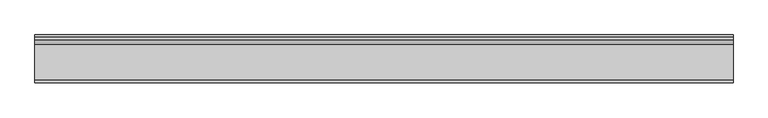
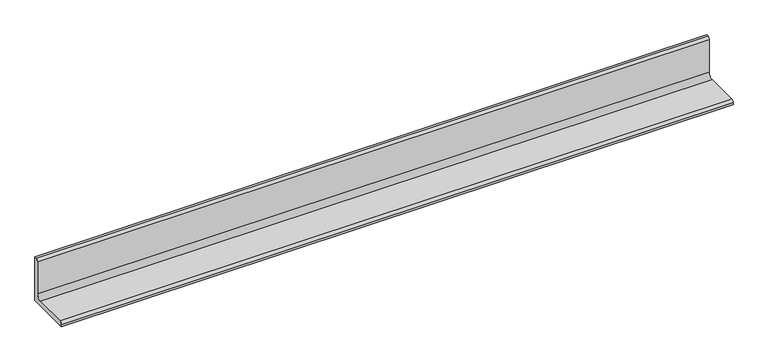
"""IFC4 building model written with IfcOpenShell, lengths in millimetres: beam geometry, NLRS_28_SF_LIB_stalen ligger hoekprofiel gelijkzijdig-AV-MMBS-SRP_gen_rsf : stalen ligger gelijkzijdig hoekprofiel LEQU_gen__150x150x15."""

from ifc_helpers import new_model, si_unit, point, frame, frame_2d, origin, place, context, project, spatial, polyline, circle_curve, trimmed, segment, composite_curve, outline, extrude, source, transform, mapped, element, save


def beam_a9a0024c(model_context):
    return source(origin(), model_context, "Body", "SweptSolid", [
        extrude(outline(composite_curve([segment(polyline([(42.5, -42.5), (-107.5, -42.5), (-107.5, -35.5)]), True, "CONTINUOUS"), segment(trimmed(circle_curve(frame_2d((-99.5, -35.5)), 8.0), [point((-107.5, -35.5))], [point((-99.5, -27.5))], False, "CARTESIAN"), True, "CONTINUOUS"), segment(polyline([(-99.5, -27.5), (11.5, -27.5)]), True, "CONTINUOUS"), segment(trimmed(circle_curve(frame_2d((11.5, -11.5)), 16.0), [point((11.5, -27.5))], [point((27.5, -11.5))], True, "CARTESIAN"), True, "CONTINUOUS"), segment(polyline([(27.5, -11.5), (27.5, 99.5)]), True, "CONTINUOUS"), segment(trimmed(circle_curve(frame_2d((35.5, 99.5)), 8.0), [point((27.5, 99.5))], [point((35.5, 107.5))], False, "CARTESIAN"), True, "CONTINUOUS"), segment(polyline([(35.5, 107.5), (42.5, 107.5), (42.5, -42.5)]), True, "CONTINUOUS")], self_intersect=False)), frame((-1095.0, 0.0, 0.0), z_axis=(1.0, 0.0, 0.0), x_axis=(0.0, 1.0, 0.0)), (0.0, 0.0, 1.0), 2190.0),
    ])


if __name__ == "__main__":
    model = new_model("IFC4")
    model_context = context("Model", 3, world=origin())
    ifc_project = project(units=[si_unit("LENGTHUNIT", "METRE", prefix="MILLI")], contexts=[model_context])
    site = spatial("IfcSite", under=ifc_project)
    building = spatial("IfcBuilding", under=site)
    placement = place(None, origin())
    beam_shape = beam_a9a0024c(model_context)
    element("IfcBeam", 1, ObjectType="NLRS_28_SF_LIB_stalen ligger hoekprofiel gelijkzijdig-AV-MMBS-SRP_gen_rsf : stalen ligger gelijkzijdig hoekprofiel LEQU_gen__150x150x15", at=placement, inside=building, context=model_context, shape_type="MappedRepresentation", body=[
        mapped(beam_shape, transform((0.0, 0.0, 0.0), x_axis=(1.0, 0.0, 0.0), y_axis=(0.0, 1.0, 0.0), z_axis=(0.0, 0.0, 1.0))),
    ])
    save(model, "model.ifc")

# Revit data of these elements
# Type "NLRS_28_SF_LIB_stalen ligger hoekprofiel gelijkzijdig-AV-MMBS-SRP_gen_rsf : stalen ligger gelijkzijdig hoekprofiel LEQU_gen__150x150x15"
#   Type IfcGUID = "2CEqVLPNH8KRN7ghwV3a1U"
#   IfcExportAs = "IfcBeamType"
#   Type Comments = "L150x150x15"
#   Model = " "
#   Manufacturer = " "
#   Fire Rating = " "
#   Description = "stalen ligger L150x150x15"
#   Assembly Code = "28.11"
#   vz = 107.5 mm
#   vy = 107.5 mm
#   tw = 15 mm
#   tf = 15 mm
#   ri = 8 mm
#   ra = 16 mm
#   d = 150 mm
#   bf = 150 mm
#   NLRS_C_lengte [instance default] = 1524 mm
#   Length [instance default] = 1524 mm
#   Structural Material = NLRS_h2_staal_gen_rsf
#   Keynote = ""
# Element 1 (IfcBeam, "NLRS_28_SF_LIB_stalen ligger hoekprofiel gelijkzijdig-AV-MMBS-SRP_gen_rsf : stalen ligger gelijkzijdig hoekprofiel LEQU_gen__150x150x15")
#   NLRS_C_lengte = 2190 mm
#   Materials on its faces: "NLRS_h2_staal_gen_rsf"
# Materials
#   "NLRS_h2_staal_gen_rsf": class "H - Metaal", colour RGB 189 187 185, transparency 0, Keynote = "h2", Manufacturer = "Revit Standards Foundation", URL = "www.revitstandards.org", Description = "staal", Cost = 0
